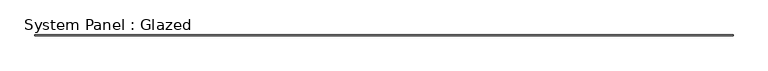
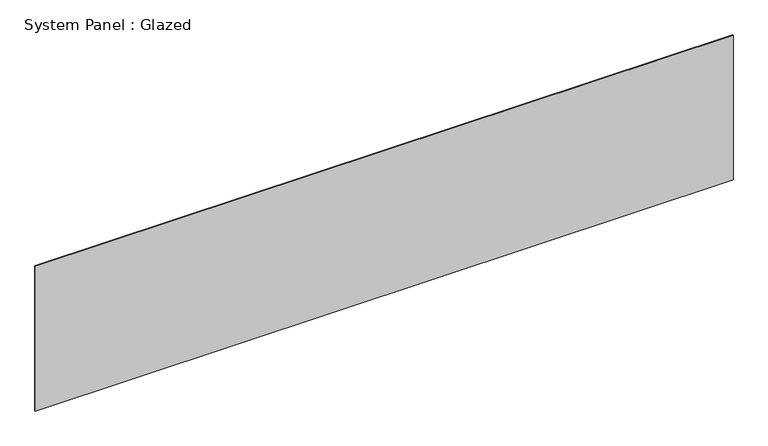
"""IFC4 building model written with IfcOpenShell, lengths in millimetres: plate geometry, System Panel : Glazed."""

from ifc_helpers import new_model, si_unit, origin, origin_with_axes, place, context, project, spatial, polyline, outline, extrude, source, transform, mapped, element, save


def system_panel_glazed_8c8fe697(model_context):
    return source(origin(), model_context, "Body", "SweptSolid", [
        extrude(outline(polyline([(13000.0, 24.5), (-13000.0, 24.5), (-13000.0, 49.5), (13000.0, 49.5), (13000.0, 24.5)])), origin_with_axes(), (0.0, 0.0, 1.0), 5700.0),
    ])


if __name__ == "__main__":
    model = new_model("IFC4")
    model_context = context("Model", 3, world=origin())
    ifc_project = project(units=[si_unit("LENGTHUNIT", "METRE", prefix="MILLI")], contexts=[model_context])
    site = spatial("IfcSite", under=ifc_project)
    building = spatial("IfcBuilding", under=site)
    placement = place(None, origin())
    system_panel_glazed_shape = system_panel_glazed_8c8fe697(model_context)
    element("IfcPlate", 1, ObjectType="System Panel : Glazed", at=placement, inside=building, context=model_context, shape_type="MappedRepresentation", body=[
        mapped(system_panel_glazed_shape, transform((0.0, 0.0, 0.0), x_axis=(1.0, 0.0, 0.0), y_axis=(0.0, 1.0, 0.0), z_axis=(0.0, 0.0, 1.0))),
    ])
    save(model, "model.ifc")

# Revit data of these elements
# Element 1 (IfcPlate, "System Panel : Glazed")
#   Materials on its faces: "Glass"
# Materials
#   "Glass": class "Glass", colour RGB 0 128 192, transparency 0.9
